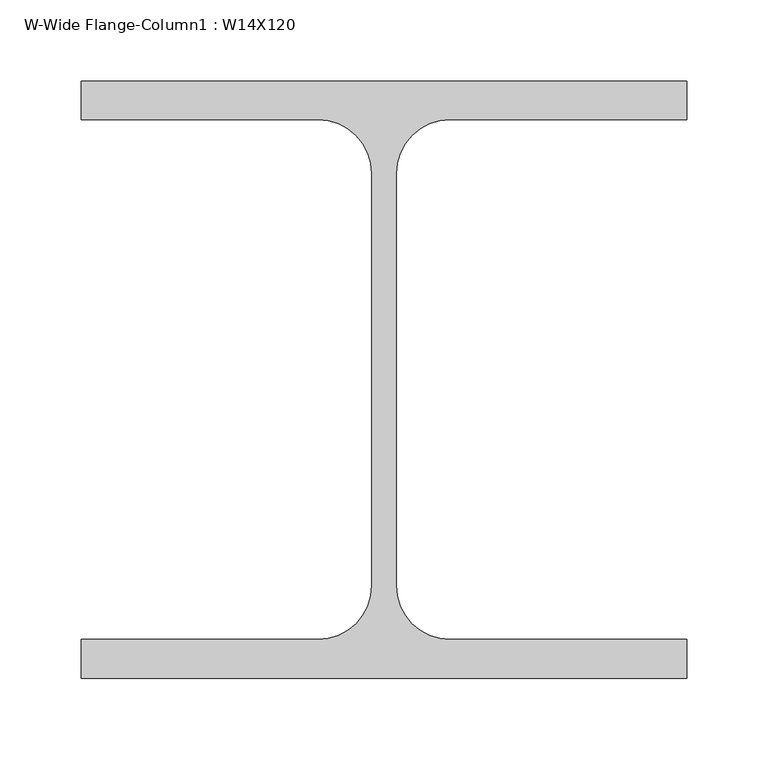
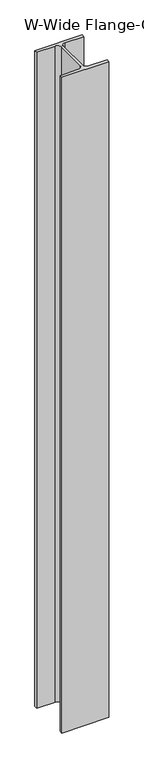
"""IFC4 building model written with IfcOpenShell, lengths in millimetres: column geometry, W-Wide Flange-Column1 : W14X120."""

from ifc_helpers import new_model, si_unit, point, frame, frame_2d, origin, place, context, project, spatial, polyline, circle_curve, trimmed, segment, composite_curve, outline, extrude, source, transform, mapped, element, save


def w_wide_flange_column1_w14x120_241bbdc2(model_context):
    return source(origin(), model_context, "Body", "SweptSolid", [
        extrude(outline(composite_curve([segment(polyline([(186.69, 184.15), (186.69, 160.274), (40.767, 160.274)]), True, "CONTINUOUS"), segment(trimmed(circle_curve(frame_2d((40.767, 127.0)), 33.274), [point((40.767, 160.274))], [point((7.493, 127.0))], True, "CARTESIAN"), True, "CONTINUOUS"), segment(polyline([(7.493, 127.0), (7.493, -127.0)]), True, "CONTINUOUS"), segment(trimmed(circle_curve(frame_2d((40.767, -127.0)), 33.274), [point((7.493, -127.0))], [point((40.767, -160.274))], True, "CARTESIAN"), True, "CONTINUOUS"), segment(polyline([(40.767, -160.274), (186.69, -160.274), (186.69, -184.15), (-186.69, -184.15), (-186.69, -160.274), (-40.767, -160.274)]), True, "CONTINUOUS"), segment(trimmed(circle_curve(frame_2d((-40.767, -127.0)), 33.274), [point((-40.767, -160.274))], [point((-7.493, -127.0))], True, "CARTESIAN"), True, "CONTINUOUS"), segment(polyline([(-7.493, -127.0), (-7.493, 127.0)]), True, "CONTINUOUS"), segment(trimmed(circle_curve(frame_2d((-40.767, 127.0)), 33.274), [point((-7.493, 127.0))], [point((-40.767, 160.274))], True, "CARTESIAN"), True, "CONTINUOUS"), segment(polyline([(-40.767, 160.274), (-186.69, 160.274), (-186.69, 184.15), (186.69, 184.15)]), True, "CONTINUOUS")], self_intersect=False)), frame((0.0, 0.0, 9144.0), z_axis=(0.0, 0.0, 1.0), x_axis=(1.0, 0.0, 0.0)), (0.0, 0.0, 1.0), 5486.4),
    ])


if __name__ == "__main__":
    model = new_model("IFC4")
    model_context = context("Model", 3, world=origin())
    ifc_project = project(units=[si_unit("LENGTHUNIT", "METRE", prefix="MILLI")], contexts=[model_context])
    site = spatial("IfcSite", under=ifc_project)
    building = spatial("IfcBuilding", under=site)
    placement = place(None, origin())
    w_wide_flange_column1_w14x120_shape = w_wide_flange_column1_w14x120_241bbdc2(model_context)
    element("IfcColumn", 1, ObjectType="W-Wide Flange-Column1 : W14X120", at=placement, inside=building, context=model_context, shape_type="MappedRepresentation", body=[
        mapped(w_wide_flange_column1_w14x120_shape, transform((0.0, 0.0, 0.0), x_axis=(1.0, 0.0, 0.0), y_axis=(0.0, 1.0, 0.0), z_axis=(0.0, 0.0, 1.0))),
    ])
    save(model, "model.ifc")

# Revit data of these elements
# Type "W-Wide Flange-Column1 : W14X120"
#   Assembly Code = "B10"
#   W = 120
#   bf = 1' - 2.7"
#   d = 1' - 2 1/2"
#   k = 0' - 2 1/4"
#   kr = 0' - 1.31"
#   tf = 0' - 0.94"
#   tw = 0' - 0.59"
#   A = 0.245139 SF
#   Structural Material [instance default] = Metal - Steel - ASTM A992
# Element 1 (IfcColumn, "W-Wide Flange-Column1 : W14X120")
#   Materials on its faces: "Metal - Steel - ASTM A992"
# Materials
#   "Metal - Steel - ASTM A992": class "Metal", colour RGB 199 199 199, transparency 0
